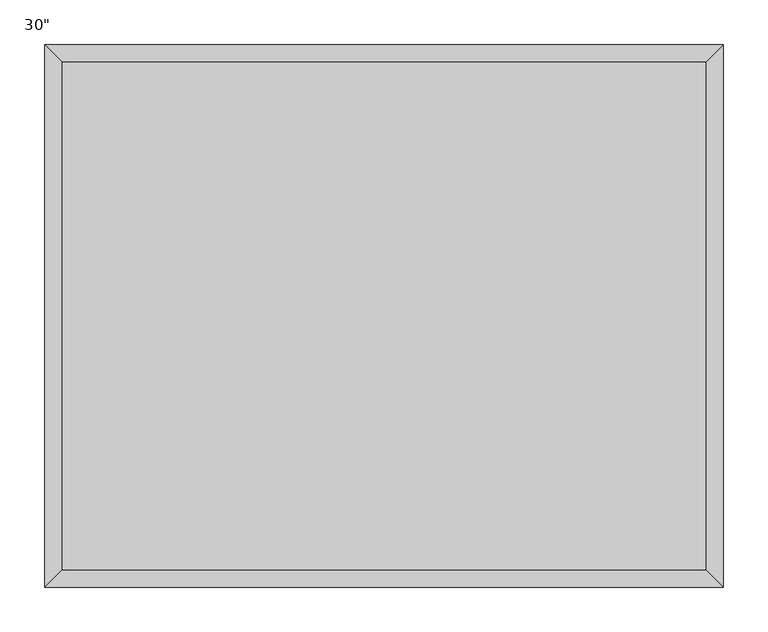
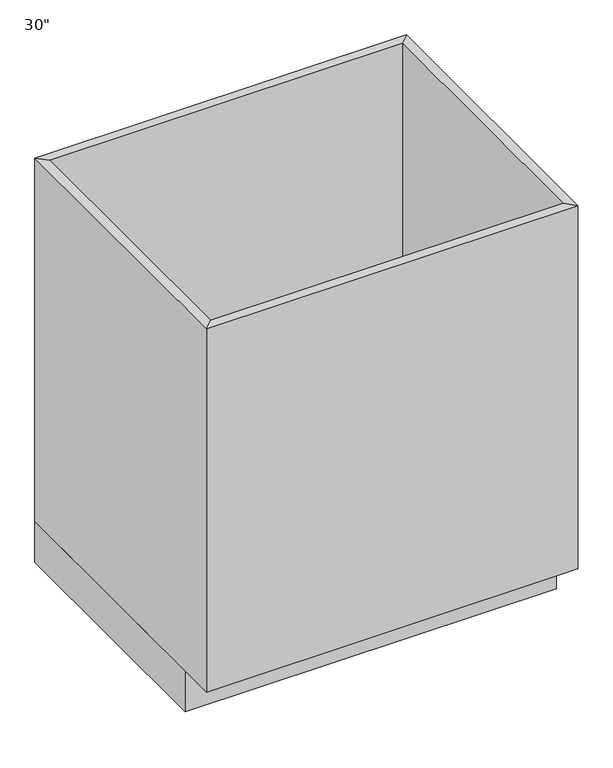
"""IFC4 building model written with IfcOpenShell, lengths in millimetres: furniture geometry."""

from ifc_helpers import new_model, si_unit, frame, origin, origin_with_axes, place, context, project, spatial, polyline, outline, extrude, faceted_brep, source, transform, mapped, element, save


def furniture_bafe1cba(model_context):
    return source(origin(), model_context, "Body", "SolidModel", [
        extrude(outline(polyline([(380.6877049, -19.05), (380.6877049, -590.55), (-343.2122951, -590.55), (-343.2122951, -19.05), (380.6877049, -19.05)])), frame((0.0, 0.0, 88.9), z_axis=(0.0, 0.0, 1.0), x_axis=(1.0, 0.0, 0.0)), (0.0, 0.0, 1.0), 19.05),
        faceted_brep([(380.6877049, -590.55, 876.3), (380.6877049, -590.55, 88.9), (-343.2122951, -590.55, 88.9), (-343.2122951, -590.55, 876.3), (399.7377049, -609.6, 876.3), (-362.2622951, -609.6, 876.3), (399.7377049, -609.6, 88.9), (-362.2622951, -609.6, 88.9), (-343.2122951, -19.05, 88.9), (-343.2122951, -19.05, 876.3), (-362.2622951, 0.0, 876.3), (-362.2622951, 0.0, 88.9), (380.6877049, -19.05, 88.9), (380.6877049, -19.05, 876.3), (399.7377049, 0.0, 876.3), (399.7377049, 0.0, 88.9)], [[[0, 1, 2, 3]], [[4, 0, 3, 5]], [[6, 4, 5, 7]], [[1, 6, 7, 2]], [[3, 2, 8, 9]], [[5, 3, 9, 10]], [[7, 5, 10, 11]], [[2, 7, 11, 8]], [[9, 8, 12, 13]], [[10, 9, 13, 14]], [[11, 10, 14, 15]], [[8, 11, 15, 12]], [[13, 12, 1, 0]], [[14, 13, 0, 4]], [[15, 14, 4, 6]], [[12, 15, 6, 1]]]),
        extrude(outline(polyline([(399.7377049, 0.0), (399.7377049, -533.4), (-362.2622951, -533.4), (-362.2622951, 0.0), (399.7377049, 0.0)])), origin_with_axes(), (0.0, 0.0, 1.0), 88.9),
    ])


if __name__ == "__main__":
    model = new_model("IFC4")
    model_context = context("Model", 3, world=origin())
    ifc_project = project(units=[si_unit("LENGTHUNIT", "METRE", prefix="MILLI")], contexts=[model_context])
    site = spatial("IfcSite", under=ifc_project)
    building = spatial("IfcBuilding", under=site)
    placement = place(None, origin())
    furniture_shape = furniture_bafe1cba(model_context)
    element("IfcFurniture", 1, ObjectType="Base Cabinet-Double Door & 1 Drawer : 30\"", at=placement, inside=building, context=model_context, shape_type="MappedRepresentation", body=[
        mapped(furniture_shape, transform((0.0, 0.0, 0.0), x_axis=(1.0, 0.0, 0.0), y_axis=(0.0, 1.0, 0.0), z_axis=(0.0, 0.0, 1.0))),
    ])
    save(model, "model.ifc")

# Revit data of these elements
# Type "Base Cabinet-Double Door & 1 Drawer : 30\""
#   Finish = "Cabinetry"
#   Depth = 2' - 0"
#   Height = 2' - 10 1/2"
#   Toe Depth = 0' - 3"
#   Toe Height = 0' - 3 1/2"
#   Width = 2' - 6"
# Element 1 (IfcFurniture, "Base Cabinet-Double Door & 1 Drawer : 30\"")
#   Materials on its faces: "Cabinet"
# Materials
#   "Cabinet": class "Wood", colour RGB 189 170 130, transparency 0, Cost = 0
